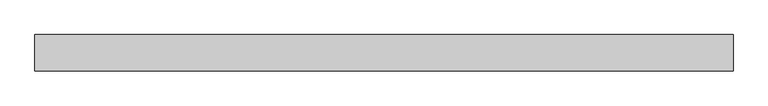
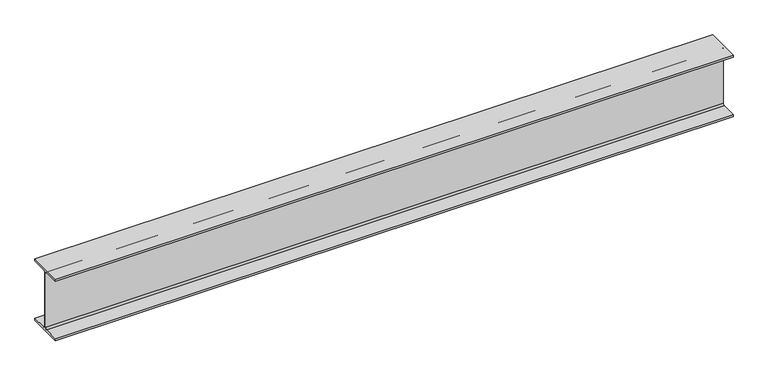
"""IFC4 building model written with IfcOpenShell, lengths in millimetres: beam geometry, Old_Steel Beam_H-KSD3502 : H_SB_ASB_H-200×200x8x12."""

from ifc_helpers import new_model, si_unit, point, frame, frame_2d, origin, place, context, project, spatial, polyline, circle_curve, trimmed, segment, composite_curve, outline, extrude, source, transform, mapped, element, save


def beam_1d8f39e2(model_context):
    return source(origin(), model_context, "Body", "SweptSolid", [
        extrude(outline(composite_curve([segment(polyline([(82.5, -141.5), (82.5, -151.7), (-82.5, -151.7), (-82.5, -141.5), (-11.9, -141.5)]), True, "CONTINUOUS"), segment(trimmed(circle_curve(frame_2d((-11.9, -132.6)), 8.9), [point((-11.9, -141.5))], [point((-3.0, -132.6))], True, "CARTESIAN"), True, "CONTINUOUS"), segment(polyline([(-3.0, -132.6), (-3.0, 132.6)]), True, "CONTINUOUS"), segment(trimmed(circle_curve(frame_2d((-11.9, 132.6)), 8.9), [point((-3.0, 132.6))], [point((-11.9, 141.5))], True, "CARTESIAN"), True, "CONTINUOUS"), segment(polyline([(-11.9, 141.5), (-82.5, 141.5), (-82.5, 151.7), (82.5, 151.7), (82.5, 141.5), (11.9, 141.5)]), True, "CONTINUOUS"), segment(trimmed(circle_curve(frame_2d((11.9, 132.6)), 8.9), [point((11.9, 141.5))], [point((3.0, 132.6))], True, "CARTESIAN"), True, "CONTINUOUS"), segment(polyline([(3.0, 132.6), (3.0, -132.6)]), True, "CONTINUOUS"), segment(trimmed(circle_curve(frame_2d((11.9, -132.6)), 8.9), [point((3.0, -132.6))], [point((11.9, -141.5))], True, "CARTESIAN"), True, "CONTINUOUS"), segment(polyline([(11.9, -141.5), (82.5, -141.5)]), True, "CONTINUOUS")], self_intersect=False)), frame((-1440.3194949, 0.0, 0.0), z_axis=(1.0, 0.0, 0.0), x_axis=(0.0, 1.0, 0.0)), (0.0, 0.0, 1.0), 3162.0635751),
    ])


if __name__ == "__main__":
    model = new_model("IFC4")
    model_context = context("Model", 3, world=origin())
    ifc_project = project(units=[si_unit("LENGTHUNIT", "METRE", prefix="MILLI")], contexts=[model_context])
    site = spatial("IfcSite", under=ifc_project)
    building = spatial("IfcBuilding", under=site)
    placement = place(None, origin())
    beam_shape = beam_1d8f39e2(model_context)
    element("IfcBeam", 1, ObjectType="Old_Steel Beam_H-KSD3502 : H_SB_ASB_H-200×200x8x12", at=placement, inside=building, context=model_context, shape_type="MappedRepresentation", body=[
        mapped(beam_shape, transform((0.0, 0.0, 0.0), x_axis=(1.0, 0.0, 0.0), y_axis=(0.0, 1.0, 0.0), z_axis=(0.0, 0.0, 1.0))),
    ])
    save(model, "model.ifc")

# Revit data of these elements
# Type "Old_Steel Beam_H-KSD3502 : H_SB_ASB_H-200×200x8x12"
#   Width = 20.0 cm
#   Web Thickness = 0.8 cm
#   Web Fillet = 1.3 cm
#   Warping Constant = 141376.0 cm⁶
#   Torsional Moment of Inertia = 26.2485 cm⁴
#   Torsional Modulus = 1.0 cm³
#   Section Area = 63.53 cm²
#   Plastic Modulus weak axis = 244.0 cm³
#   Plastic Modulus strong axis = 525.0 cm³
#   Perimeter = 1.16 m²/m
#   Nominal Weight = 49.90 kgf/m
#   Moment of Inertia weak axis = 1600.00 cm⁴
#   Moment of Inertia strong axis = 4720.00 cm⁴
#   Height = 20.0 cm
#   Flange Thickness = 1.2 cm
#   Elastic Modulus weak axis = 160.0 cm³
#   Elastic Modulus strong axis = 472.0 cm³
#   Centroid Vertical = 10.0 cm
#   Centroid Horizontal = 10.0 cm
#   Length [instance default] = 1.5240 m
#   Structural Material [instance default] = Steel, 45-345
#   Assembly Code = ""
# Element 1 (IfcBeam, "Old_Steel Beam_H-KSD3502 : H_SB_ASB_H-200×200x8x12")
#   Structural Material = none
# Materials
#   "Steel, 45-345": class "Metal", colour RGB 189 187 185, transparency 0, Description = "Steel 345 MPa", Cost = 0
